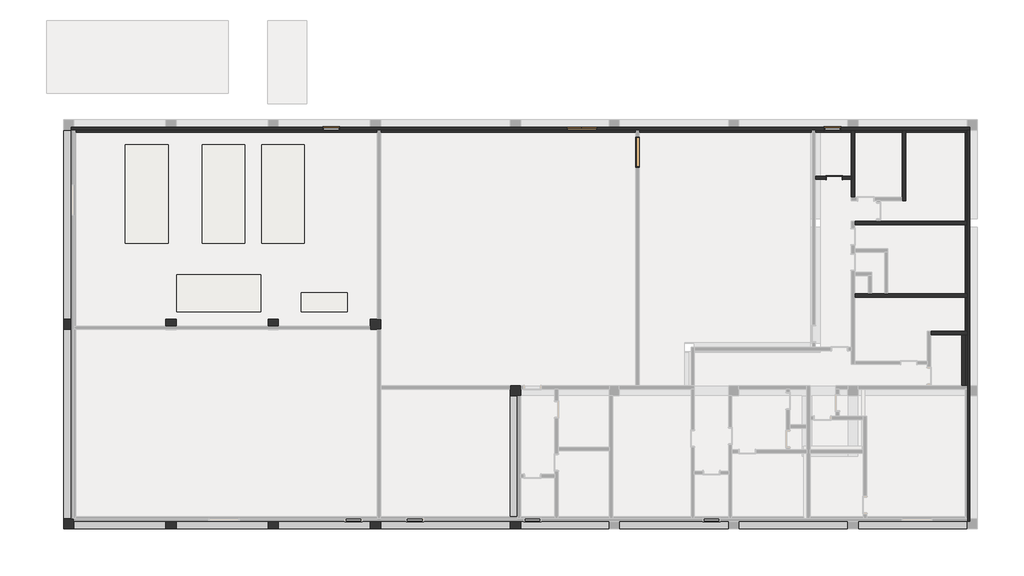
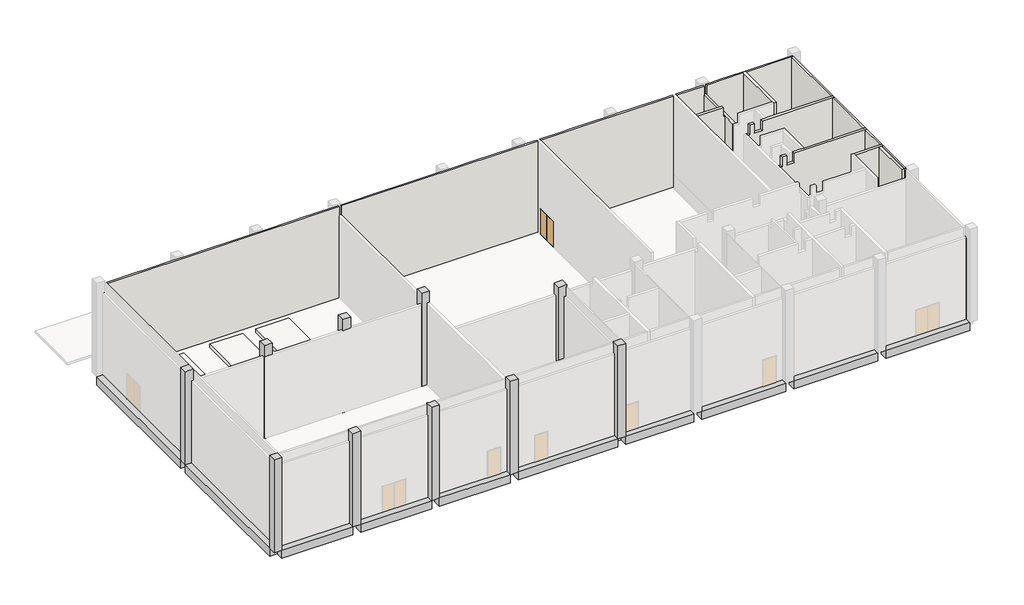
# One storey, part 3 of 4: 19 walls, 10 columns, 5 doors, 5 slabs, 3 beams.
# Revit data of these elements (continued)
# Type "H_SF_AR B01_EQ Fdn_EF4 4900x2300x200" (continued)
#   Type Comments = "EQUIP. FDN"
#   Type Mark = ""
#   Layers, outside or top first: 200 mm "00_Concrete_Reinf. Conc." (function 1)
# Type "H_SF_AR B01_EQ Fdn_EF5 2700x1100x200"
#   Type Comments = "EQUIP. FDN"
#   Type Mark = ""
#   Layers, outside or top first: 200 mm "00_Concrete_Reinf. Conc." (function 1)
# Type "H_WA_AR B02_Ext Wall RC-AG_EW5"
#   Type Comments = "AG"
#   Type Mark = "W1"
#   H_Rebar Ratio = 0.12
#   Layers, outside or top first: 0 mm no material (function 100); 0 mm no material (function 100); 150 mm no material (function 1); 0 mm no material (function 100); 0 mm no material (function 100); 0 mm no material (function 100)
# Type "H_WA_AR B02_Int Wall MA_IW1 T200"
#   Type Comments = ""
#   Layers, outside or top first: 200 mm "00_Masonry_Conc. Block" (function 1)
# Type "H_WA_AR B02_Ext Wall DY-IN_EW1_VB"
#   Type Comments = "구조_콘크리트"
#   Layers, outside or top first: 126 mm "Rock Wool" (function 1)
# Elements 1, 2 (IfcBeam, "RC Beam_Rectangular : H_SB_AR S16_TG-UG_TG1 600x650")
#   Comments = ""
#   hec_material3 = none
#   hec_material2 = none
#   hec_material1 = none
#   Structural Material = 00_Concrete_Reinf. Conc.
#   Phase Created = New Construction
#   Materials on its faces: "00_Concrete_Reinf. Conc."
# Element 3 (IfcBeam, "RC Beam_Rectangular : H_SB_AR S16_TG-UG_TG1 600x650")
#   hec_material3 = none
#   hec_material2 = none
#   hec_material1 = none
#   Structural Material = 00_Concrete_Reinf. Conc.
#   Phase Created = New Construction
#   Materials on its faces: "00_Concrete_Reinf. Conc."
# Element 4 (IfcColumn, "RC_Column_Rectangular : H_SC_AR S15_RC Col-AG_C1 600x600")
#   IfcGUID = "23HYWPttL4pwJG8hldAB8o"
#   Comments = ""
#   Phase Created = New Construction
#   Materials on its faces: "00_Concrete_Reinf. Conc."
# Elements 5, 6, 7, 8, 9, 10, 11, 12 (IfcColumn, "RC_Column_Rectangular : H_SC_AR S15_RC Col-AG_C1 600x600")
#   Comments = ""
#   Phase Created = New Construction
#   Materials on its faces: "00_Concrete_Reinf. Conc."
# Element 13 (IfcColumn, "RC_Column_Rectangular : H_SC_AR S15_RC Col-AG_C2 600x600 2")
#   IfcGUID = "23HYWPttL4pwJG8hldABIl"
#   Comments = ""
#   Phase Created = New Construction
#   Materials on its faces: "00_Concrete_Reinf. Conc."
# Elements 14, 15 (IfcDoor, "Double Door_Steel : H_DR_AR B12_Door_Double FSD 02")
#   Frame Material = "ST"
#   H_Door Style Name = "Steel Door_Double_Normal_Fire Rating"
#   H_Door_Leaf = "ST"
#   H_Door_Vision = "-"
#   H_Door_Panic = "-"
#   H_Door_Style Remark = ""
#   H_Door_Type = "B1"
#   H_Door_Louver = "-"
#   H_Door Style No = 212_FSD_DD_N_F
#   Phase Created = New Construction
# Elements 16, 18 (IfcDoor, "Single Door_Steel : H_DR_AR B12_Door_Single FSD 01")
#   Frame Material = "ST"
#   H_Door Style Name = "Steel Door_Single_Normal_Fire Rating"
#   H_Door_Leaf = "ST"
#   H_Door_Vision = "-"
#   H_Door_Panic = "-"
#   H_Door_Style Remark = ""
#   H_Door_Type = "A1"
#   H_Door_Louver = "-"
#   H_Door Style No = 112_FSD_SD_N_F
#   Phase Created = New Construction
# Element 17 (IfcDoor, "Single Door_Steel : H_DR_AR B12_Door_Single FSD 01")
#   Frame Material = "ST"
#   H_Door Style Name = "Steel Door_Single_Panic Bar_Fire Rating"
#   H_Door_Leaf = "ST"
#   H_Door_Vision = "-"
#   H_Door_Panic = "O"
#   H_Door_Style Remark = ""
#   H_Door_Type = "A1"
#   H_Door_Louver = "-"
#   H_Door Style No = 132_FSD_SD_P_F
#   Phase Created = New Construction
# Elements 19, 20, 21 (IfcSlab, "H_SF_AR B01_EQ Fdn_EF3 2500x5800x300")
#   Comments = ""
#   Mark = "EF3"
#   Height Offset From Level = 300 mm
#   built-in parameter 1001954 = 1
#   Phase Created = New Construction
#   Materials on its faces: "00_Concrete_Reinf. Conc."
# Element 22 (IfcSlab, "H_SF_AR B01_EQ Fdn_EF4 4900x2300x200")
#   Comments = ""
#   Mark = "EF4"
#   Height Offset From Level = 200 mm
#   built-in parameter 1001954 = 1
#   Phase Created = New Construction
#   Materials on its faces: "00_Concrete_Reinf. Conc."
# Element 23 (IfcSlab, "H_SF_AR B01_EQ Fdn_EF5 2700x1100x200")
#   Comments = ""
#   Mark = "EF5"
#   Height Offset From Level = 200 mm
#   built-in parameter 1001954 = 1
#   Phase Created = New Construction
#   Materials on its faces: "00_Concrete_Reinf. Conc."
# Elements 24, 25 (IfcWall, "H_WA_AR B02_Ext Wall RC-AG_EW5")
#   H_Wall Style Name = "Concrete Wall+Acrylic Emulsion Paint on Fair Faced Concrete+Insulation"
#   H_Wall_Style Remark = ""
#   Top Offset = 0 mm
#   Base Offset = 0 mm
#   wall height = 7500.038 mm
#   H_Wall Style No = EW512A_CO
#   Phase Created = New Construction
#   Base Constraint = TOC(GF)
#   Top Constraint = TOC
#   Materials on its faces: "00_Concrete_Reinf. Conc."
# Elements 26, 27, 28, 29, 30, 31, 32 (IfcWall, "H_WA_AR B02_Int Wall MA_IW1 T200")
#   H_Wall Style Name = "Block Wall"
#   H_Wall_Style Remark = ""
#   Top Offset = 0 mm
#   Base Offset = 0 mm
#   wall height = 7500.038 mm
#   H_Wall Style No = IW211_BL
#   Phase Created = New Construction
#   Base Constraint = TOC(GF)
#   Top Constraint = TOC
#   Materials on its faces: "00_Masonry_Conc. Block"
# Elements 33, 34, 35, 36, 37, 38, 39, 40, 41, 42 (IfcWall, "H_WA_AR B02_Ext Wall DY-IN_EW1_VB")
#   Top Offset = 0 mm
#   Base Offset = 0 mm
#   wall height = 7500.038 mm
#   Phase Created = New Construction
#   Base Constraint = TOC(GF)
#   Top Constraint = TOC
#   Materials on its faces: "Rock Wool"
# Materials
#   "00_Concrete_Reinf. Conc.": class "Concrete", colour RGB 176 176 176, transparency 0, Description = "Reinf. Conc.", Cost = 0, Image = Concrete.Cast-In-Place.Flat.Polished.Grey.jpg
#   "00_Masonry_Conc. Block": class "Concrete", colour RGB 180 180 180, transparency 0, Description = "Conc. Block", Cost = 0, Image = Brick_Uniform_12inch_Running_Gray.png
#   "Rock Wool": class "Generic", colour RGB 120 120 120, transparency 0, Description = "Rock Wool", Cost = 0
